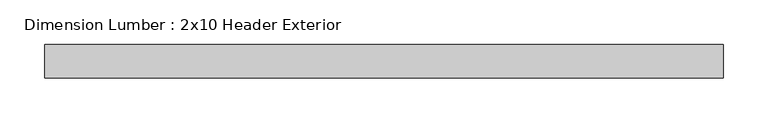
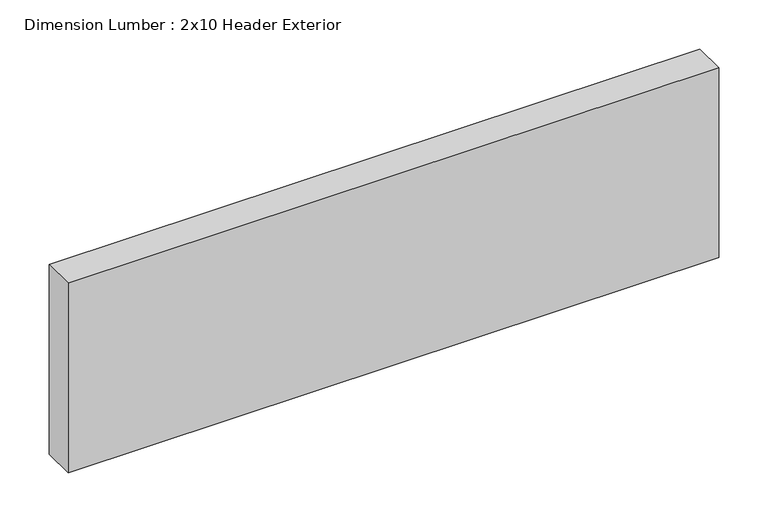
"""IFC4 building model written with IfcOpenShell, lengths in millimetres: beam geometry, Dimension Lumber : 2x10 Header Exterior."""

from ifc_helpers import new_model, si_unit, frame, origin, place, context, project, spatial, polyline, outline, extrude, source, transform, mapped, element, save


def dimension_lumber_2x10_header_exterior_1f1296b6(model_context):
    return source(origin(), model_context, "Body", "SweptSolid", [
        extrude(outline(polyline([(468.709375, 19.05), (468.709375, -19.05), (-293.290625, -19.05), (-293.290625, 19.05), (468.709375, 19.05)])), frame((0.0, 0.0, -117.475), z_axis=(0.0, 0.0, 1.0), x_axis=(1.0, 0.0, 0.0)), (0.0, 0.0, 1.0), 234.95),
    ])


if __name__ == "__main__":
    model = new_model("IFC4")
    model_context = context("Model", 3, world=origin())
    ifc_project = project(units=[si_unit("LENGTHUNIT", "METRE", prefix="MILLI")], contexts=[model_context])
    site = spatial("IfcSite", under=ifc_project)
    building = spatial("IfcBuilding", under=site)
    placement = place(None, origin())
    dimension_lumber_2x10_header_exterior_shape = dimension_lumber_2x10_header_exterior_1f1296b6(model_context)
    element("IfcBeam", 1, ObjectType="Dimension Lumber : 2x10 Header Exterior", at=placement, inside=building, context=model_context, shape_type="MappedRepresentation", body=[
        mapped(dimension_lumber_2x10_header_exterior_shape, transform((0.0, 0.0, 0.0), x_axis=(1.0, 0.0, 0.0), y_axis=(0.0, 1.0, 0.0), z_axis=(0.0, 0.0, 1.0))),
    ])
    save(model, "model.ifc")

# Revit data of these elements
# Type "Dimension Lumber : 2x10 Header Exterior"
#   Assembly Code = "B10"
#   A = 0.0963889 SF
#   Length [instance default] = 5' - 0"
#   b = 0' - 1 1/2"
#   d = 0' - 9 1/4"
#   Structural Material [instance default] = Softwood, Lumber
# Element 1 (IfcBeam, "Dimension Lumber : 2x10 Header Exterior")
#   Structural Material = Douglas Fir #2
#   Materials on its faces: "Douglas Fir #2"
# Materials
#   "Softwood, Lumber": class "Wood", colour RGB 223 192 134, transparency 0, Description = "Pinus Echinata", Cost = 0
#   "Douglas Fir #2": class "Wood", colour RGB 223 192 134, transparency 0, Description = "Pinus Echinata", Cost = 0
